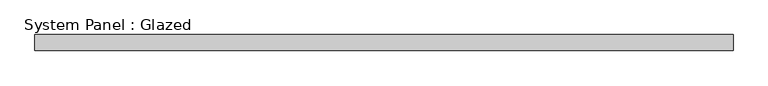
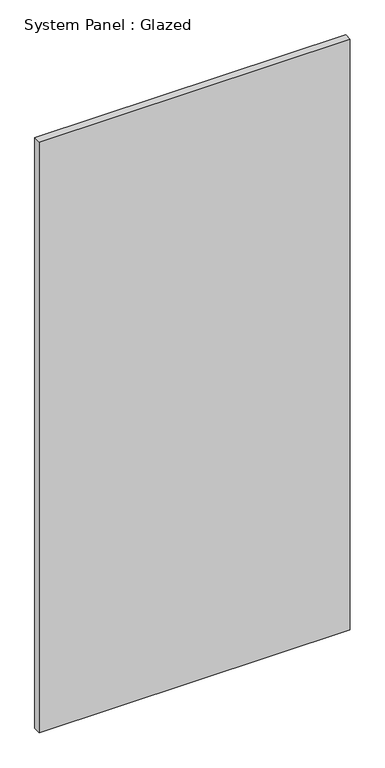
"""IFC4 building model written with IfcOpenShell, lengths in millimetres: plate geometry, System Panel : Glazed."""

import ifcopenshell
import ifcopenshell.guid

model = None  # the IFC model being written
_history = None  # IfcOwnerHistory: only IFC2X3 demands one
_inside = {}  # id of a spatial element -> (the spatial element, [elements in it])
_under = {}  # id of a project, library or spatial element -> (it, [spatial elements below it])
_declared = {}  # id of a project -> (the project, [libraries it declares])
_typed = {}  # id of a type object -> (the type object, [elements of that type])
_made_of = {}  # id of a material, layer set ... -> (it, [elements and type objects made of it])


def new_model(schema):
    """Start an empty IFC model of exactly this schema.

    Asked for "IFC4X3", IfcOpenShell would pick the latest addendum, in which some entities
    have other attributes; the version numbers below select the first issue.
    IFC2X3 requires an IfcOwnerHistory on every rooted entity: one is made here for all.
    """
    global model, _history
    if schema == "IFC4X3":
        model = ifcopenshell.file(schema_version=(4, 3, 0, 0))
    else:
        model = ifcopenshell.file(schema=schema)
    _inside.clear()
    _under.clear()
    _declared.clear()
    _typed.clear()
    _made_of.clear()
    _history = None
    if model.schema == "IFC2X3":
        org = make("IfcOrganization", Name="unknown")
        user = make(
            "IfcPersonAndOrganization",
            ThePerson=make("IfcPerson", FamilyName="unknown"),
            TheOrganization=org,
        )
        app = make(
            "IfcApplication",
            ApplicationDeveloper=org,
            Version="unknown",
            ApplicationFullName="unknown",
            ApplicationIdentifier="unknown",
        )
        _history = make(
            "IfcOwnerHistory",
            OwningUser=user,
            OwningApplication=app,
            ChangeAction="ADDED",
            CreationDate=0,
        )
    return model


def make(cls, **values):
    """One entity of the class cls with the attributes given. An attribute that is None is left unset."""
    return model.create_entity(
        cls, **{name: value for name, value in values.items() if value is not None}
    )


def rooted(cls, **values):
    """An entity with a GlobalId (a new one), such as an element, a storey or a relation."""
    return make(cls, GlobalId=ifcopenshell.guid.new(), OwnerHistory=_history, **values)


def si_unit(unit_type, name, prefix=None):
    """IfcSIUnit, for example si_unit("LENGTHUNIT", "METRE", prefix="MILLI")."""
    return make("IfcSIUnit", UnitType=unit_type, Prefix=prefix, Name=name)


def assignment(units):
    """IfcUnitAssignment: the units of a project."""
    return None if units is None else make("IfcUnitAssignment", Units=units)


def point(xyz):
    """IfcCartesianPoint."""
    return None if xyz is None else make("IfcCartesianPoint", Coordinates=xyz)


def direction(xyz):
    """IfcDirection."""
    return None if xyz is None else make("IfcDirection", DirectionRatios=xyz)


def frame(location, z_axis=None, x_axis=None):
    """IfcAxis2Placement3D, a coordinate frame: its origin and axes. An axis left out is left unset."""
    return make(
        "IfcAxis2Placement3D",
        Location=point(location),
        Axis=direction(z_axis),
        RefDirection=direction(x_axis),
    )


def origin():
    """The frame at (0, 0, 0) with its axes left unset."""
    return frame((0.0, 0.0, 0.0))


def origin_with_axes():
    """The frame at (0, 0, 0) with the z axis (0, 0, 1) and the x axis (1, 0, 0) written out."""
    return frame((0.0, 0.0, 0.0), z_axis=(0.0, 0.0, 1.0), x_axis=(1.0, 0.0, 0.0))


def place(relative_to, where):
    """IfcLocalPlacement: puts the frame where relative to a parent placement (None: the world)."""
    return make(
        "IfcLocalPlacement", PlacementRelTo=relative_to, RelativePlacement=where
    )


def context(
    kind, dimensions, precision=None, world=None, true_north=None, identifier=None
):
    """IfcGeometricRepresentationContext, for example the 3D "Model" context."""
    return make(
        "IfcGeometricRepresentationContext",
        ContextIdentifier=identifier,
        ContextType=kind,
        CoordinateSpaceDimension=dimensions,
        Precision=precision,
        WorldCoordinateSystem=world,
        TrueNorth=true_north,
    )


def project(units=None, contexts=None):
    """IfcProject with its units and contexts."""
    return rooted(
        "IfcProject",
        Name="project",
        RepresentationContexts=contexts,
        UnitsInContext=assignment(units),
    )


def spatial(cls, under=None, at=None, **own):
    """A site, building, storey or space (cls), placed at a placement, below another one or the project."""
    s = rooted(cls, ObjectPlacement=at, **own)
    if under is not None:
        _under.setdefault(under.id(), (under, []))[1].append(s)
    return s


def polyline(points):
    """IfcPolyline through the points."""
    return make("IfcPolyline", Points=[point(p) for p in points])


def outline(outer, holes=None, kind="AREA"):
    """IfcArbitraryClosedProfileDef: a profile drawn as a closed curve; with holes, ...WithVoids."""
    if holes is None:
        return make("IfcArbitraryClosedProfileDef", ProfileType=kind, OuterCurve=outer)
    return make(
        "IfcArbitraryProfileDefWithVoids",
        ProfileType=kind,
        OuterCurve=outer,
        InnerCurves=holes,
    )


def extrude(swept, where, along, depth):
    """IfcExtrudedAreaSolid: the profile swept, set in the frame where, extruded along a direction by depth."""
    return make(
        "IfcExtrudedAreaSolid",
        SweptArea=swept,
        Position=where,
        ExtrudedDirection=direction(along),
        Depth=depth,
    )


def shape(context_of_items, identifier, shape_type, items):
    """IfcShapeRepresentation: the items that make up one representation, for example the "Body"."""
    return make(
        "IfcShapeRepresentation",
        ContextOfItems=context_of_items,
        RepresentationIdentifier=identifier,
        RepresentationType=shape_type,
        Items=items,
    )


def source(mapping_origin, context_of_items, identifier, shape_type, items):
    """IfcRepresentationMap: a shape defined once, which mapped items show again and again."""
    return make(
        "IfcRepresentationMap",
        MappingOrigin=mapping_origin,
        MappedRepresentation=shape(context_of_items, identifier, shape_type, items),
    )


def transform(
    local_origin,
    x_axis=None,
    y_axis=None,
    z_axis=None,
    scale=None,
    scale2=None,
    scale3=None,
    uniform=True,
):
    """IfcCartesianTransformationOperator3D, or its non-uniform kind. x_axis, y_axis, z_axis: its Axis1, 2, 3."""
    if uniform:
        return make(
            "IfcCartesianTransformationOperator3D",
            Axis1=direction(x_axis),
            Axis2=direction(y_axis),
            LocalOrigin=point(local_origin),
            Scale=scale,
            Axis3=direction(z_axis),
        )
    return make(
        "IfcCartesianTransformationOperator3DnonUniform",
        Axis1=direction(x_axis),
        Axis2=direction(y_axis),
        LocalOrigin=point(local_origin),
        Scale=scale,
        Axis3=direction(z_axis),
        Scale2=scale2,
        Scale3=scale3,
    )


def mapped(mapping_source, mapping_target):
    """IfcMappedItem: shows the shape of a source again, moved by a transform."""
    return make(
        "IfcMappedItem", MappingSource=mapping_source, MappingTarget=mapping_target
    )


def made_of(thing, what):
    """Note that an element or type object is made of a material, layer set ...; save() writes the relation."""
    if what is not None:
        _made_of.setdefault(what.id(), (what, []))[1].append(thing)
    return thing


def element(
    cls,
    number,
    at=None,
    inside=None,
    cuts=None,
    type_object=None,
    material=None,
    context=None,
    identifier="Body",
    shape_type=None,
    held_by="IfcProductDefinitionShape",
    body=None,
    shapes=None,
    **own,
):
    """One element of the class cls, such as IfcWall. Its Tag is "e" and its number.

    at: its placement. inside: the storey or other place that contains it. cuts: it is an
    opening in that element (IfcRelVoidsElement). A single representation is given by context,
    identifier, shape_type and body (its items); several are given by shapes. held_by: the class
    of the entity that holds the representations. save() writes the other relations.
    """
    e = rooted(cls, Tag="e%d" % number, ObjectPlacement=at, **own)
    if body is not None:
        shapes = [shape(context, identifier, shape_type, body)]
    if shapes is not None:
        e.Representation = make(held_by, Representations=shapes)
    if inside is not None:
        _inside.setdefault(inside.id(), (inside, []))[1].append(e)
    if cuts is not None:
        rooted(
            "IfcRelVoidsElement", RelatingBuildingElement=cuts, RelatedOpeningElement=e
        )
    if type_object is not None:
        _typed.setdefault(type_object.id(), (type_object, []))[1].append(e)
    return made_of(e, material)


def aggregate(whole, parts):
    """IfcRelAggregates: a whole, such as a stair, and the parts it consists of."""
    return rooted("IfcRelAggregates", RelatingObject=whole, RelatedObjects=parts)


def save(model, path):
    """Write the relations noted so far, then the file.

    IfcRelAggregates (storeys below a building ...), IfcRelContainedInSpatialStructure (elements
    in a storey), IfcRelDefinesByType, IfcRelAssociatesMaterial and IfcRelDeclares: one each for
    every whole, place, type object, material and project.
    """
    for whole, parts in _under.values():
        aggregate(whole, parts)
    for where, things in _inside.values():
        rooted(
            "IfcRelContainedInSpatialStructure",
            RelatedElements=things,
            RelatingStructure=where,
        )
    for kind, things in _typed.values():
        rooted("IfcRelDefinesByType", RelatedObjects=things, RelatingType=kind)
    for what, things in _made_of.values():
        rooted("IfcRelAssociatesMaterial", RelatedObjects=things, RelatingMaterial=what)
    for by, libraries in _declared.values():
        rooted("IfcRelDeclares", RelatingContext=by, RelatedDefinitions=libraries)
    model.write(path)


def system_panel_glazed_578ed88e(model_context):
    return source(origin(), model_context, "Body", "SweptSolid", [
        extrude(outline(polyline([(551.965768, -44.45), (-551.965768, -44.45), (-551.965768, -19.05), (551.965768, -19.05), (551.965768, -44.45)])), origin_with_axes(), (0.0, 0.0, 1.0), 2216.15),
    ])


if __name__ == "__main__":
    model = new_model("IFC4")
    model_context = context("Model", 3, world=origin())
    ifc_project = project(units=[si_unit("LENGTHUNIT", "METRE", prefix="MILLI")], contexts=[model_context])
    site = spatial("IfcSite", under=ifc_project)
    building = spatial("IfcBuilding", under=site)
    placement = place(None, origin())
    system_panel_glazed_shape = system_panel_glazed_578ed88e(model_context)
    element("IfcPlate", 1, ObjectType="System Panel : Glazed", at=placement, inside=building, context=model_context, shape_type="MappedRepresentation", body=[
        mapped(system_panel_glazed_shape, transform((0.0, 0.0, 0.0), x_axis=(1.0, 0.0, 0.0), y_axis=(0.0, 1.0, 0.0), z_axis=(0.0, 0.0, 1.0))),
    ])
    save(model, "model.ifc")

# Revit data of these elements
# Type "System Panel : Glazed"
#   Construction Type Id = "GSP4R"
#   Analytic Construction = "1/8 in Pilkington single glazing"
#   Visual Light Transmittance = 0.9
#   Solar Heat Gain Coefficient = 0.86
#   Heat Transfer Coefficient (U) = 1.18115 BTU/(h·ft²·°F)
#   Define Thermal Properties by = 1
# Element 1 (IfcPlate, "System Panel : Glazed")
#   Materials on its faces: "Glass"
# Materials
#   "Glass": class "Glass", colour RGB 0 128 192, transparency 0.75, Description = "Soda Lime Glass", Cost = 0
